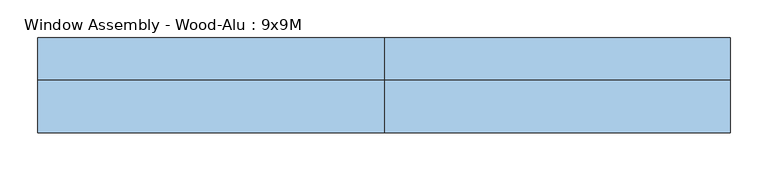
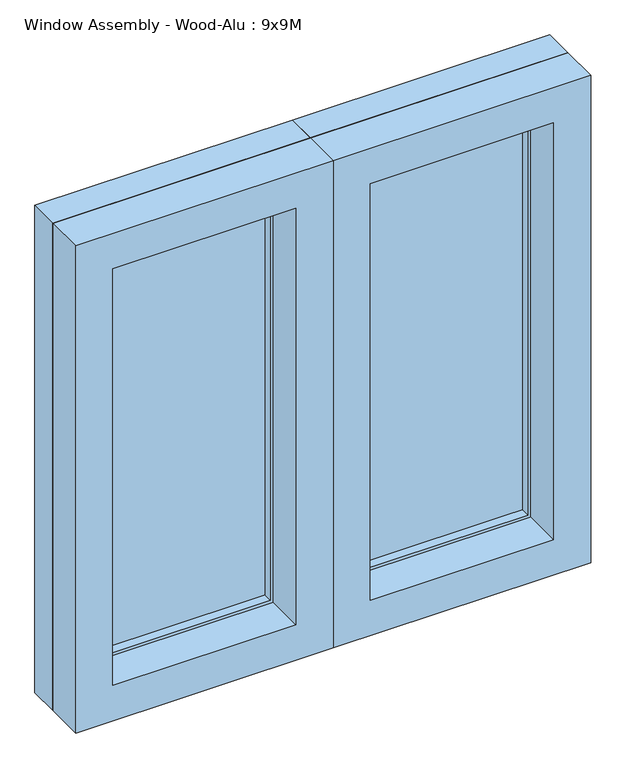
"""IFC4 building model written with IfcOpenShell, lengths in millimetres: window geometry, Window Assembly - Wood-Alu : 9x9M."""

from ifc_helpers import new_model, si_unit, frame, origin, place, context, project, spatial, polyline, outline, extrude, source, transform, mapped, element, save


def window_assembly_wood_alu_9x9m_7c5911af(model_context):
    return source(origin(), model_context, "Body", "SweptSolid", [
        extrude(outline(polyline([(1712.0, 0.0), (1712.0, -456.0), (800.0, -456.0), (800.0, 0.0), (1712.0, 0.0)]), holes=[polyline([(1641.0, -385.0), (1641.0, -71.0), (871.0, -71.0), (871.0, -385.0), (1641.0, -385.0)])]), frame((0.0, 129.0, 0.0), z_axis=(0.0, 1.0, 0.0), x_axis=(0.0, 0.0, 1.0)), (0.0, 0.0, 1.0), 55.0),
        extrude(outline(polyline([(1712.0, 0.0), (1712.0, -456.0), (800.0, -456.0), (800.0, 0.0), (1712.0, 0.0)]), holes=[polyline([(1646.0, -390.0), (1646.0, -66.0), (866.0, -66.0), (866.0, -390.0), (1646.0, -390.0)])]), frame((0.0, 59.0, 0.0), z_axis=(0.0, 1.0, 0.0), x_axis=(0.0, 0.0, 1.0)), (0.0, 0.0, 1.0), 70.0),
        extrude(outline(polyline([(-385.0, 145.5), (-385.0, 167.5), (-71.0, 167.5), (-71.0, 145.5), (-385.0, 145.5)])), frame((0.0, 0.0, 871.0), z_axis=(0.0, 0.0, 1.0), x_axis=(1.0, 0.0, 0.0)), (0.0, 0.0, 1.0), 770.0),
        extrude(outline(polyline([(1712.0, 0.0), (800.0, 0.0), (800.0, 456.0), (1712.0, 456.0), (1712.0, 0.0)]), holes=[polyline([(1641.0, 385.0), (871.0, 385.0), (871.0, 71.0), (1641.0, 71.0), (1641.0, 385.0)])]), frame((0.0, 129.0, 0.0), z_axis=(0.0, 1.0, 0.0), x_axis=(0.0, 0.0, 1.0)), (0.0, 0.0, 1.0), 55.0),
        extrude(outline(polyline([(1712.0, 0.0), (800.0, 0.0), (800.0, 456.0), (1712.0, 456.0), (1712.0, 0.0)]), holes=[polyline([(1646.0, 390.0), (866.0, 390.0), (866.0, 66.0), (1646.0, 66.0), (1646.0, 390.0)])]), frame((0.0, 59.0, 0.0), z_axis=(0.0, 1.0, 0.0), x_axis=(0.0, 0.0, 1.0)), (0.0, 0.0, 1.0), 70.0),
        extrude(outline(polyline([(385.0, 145.5), (71.0, 145.5), (71.0, 167.5), (385.0, 167.5), (385.0, 145.5)])), frame((0.0, 0.0, 871.0), z_axis=(0.0, 0.0, 1.0), x_axis=(1.0, 0.0, 0.0)), (0.0, 0.0, 1.0), 770.0),
    ])


if __name__ == "__main__":
    model = new_model("IFC4")
    model_context = context("Model", 3, world=origin())
    ifc_project = project(units=[si_unit("LENGTHUNIT", "METRE", prefix="MILLI")], contexts=[model_context])
    site = spatial("IfcSite", under=ifc_project)
    building = spatial("IfcBuilding", under=site)
    placement = place(None, origin())
    window_assembly_wood_alu_9x9m_shape = window_assembly_wood_alu_9x9m_7c5911af(model_context)
    element("IfcWindow", 1, ObjectType="Window Assembly - Wood-Alu : 9x9M", at=placement, inside=building, context=model_context, shape_type="MappedRepresentation", body=[
        mapped(window_assembly_wood_alu_9x9m_shape, transform((0.0, 0.0, 0.0), x_axis=(1.0, 0.0, 0.0), y_axis=(0.0, 1.0, 0.0), z_axis=(0.0, 0.0, 1.0))),
    ])
    save(model, "model.ifc")

# Revit data of these elements
# Type "Window Assembly - Wood-Alu : 9x9M"
#   Type Mark = "51"
#   Creator Organization [instance default] = "© Danish Educational Content"
#   Creator Name [instance default] = "© Erik Falck Jørgensen"
#   Creator Build [instance default] = "2017.0801.0"
#   Analytic Construction = "<None>"
#   length#5 = 132 mm
#   length#6 = 125 mm
#   length#7 = 456 mm
#   length#3 = 71 mm
#   length#8 = 912 mm
#   length#4 = 125 mm
#   Seal Width = 12 mm
#   length#2 = 66 mm
#   length#1 = 0 mm
#   Rough Width = 912 mm
#   Rough Height = 912 mm
#   Rebate Depth = 50 mm
#   Joining Width = 8 mm
#   Joining Depth = 62 mm
#   Height = 888 mm
#   Glass Thickness = 22 mm
#   Frame Width = 55 mm
#   Frame Depth = 55 mm
#   Exterior Direction [instance default] = 0.00°
#   Element Width = 440 mm
#   Default Sill Height = 800 mm
#   Width = 888 mm
#   Case Width = 50 mm
#   Case Depth = 70 mm
#   Sealing = no
#   Hinging = yes
#   Wall Closure = 1
#   Above Cutplane [instance default] = no
#   Glass = none
#   Frame/Mullion = none
#   Case/Transom = none
#   Assembly Code = ""
# Element 1 (IfcWindow, "Window Assembly - Wood-Alu : 9x9M")
#   Materials on its faces: "Default Frame/Mullion (Interior/Exterior)", "Glass"
# Materials
#   "Default Frame/Mullion (Interior/Exterior)": class "Generic", colour RGB 205 205 205, transparency 0, Description = "Udefineret karm/ramme materiale", Cost = 0
#   "Glass": class "Glass", colour RGB 180 200 255, transparency 0.75, Description = "Generisk glas", Cost = 0
